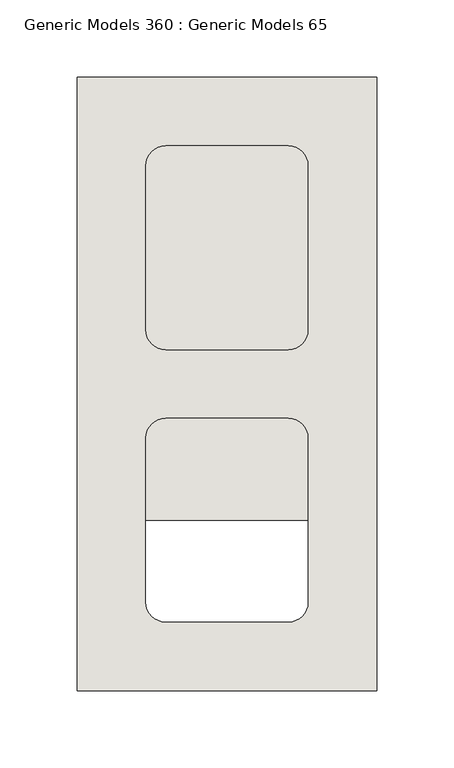
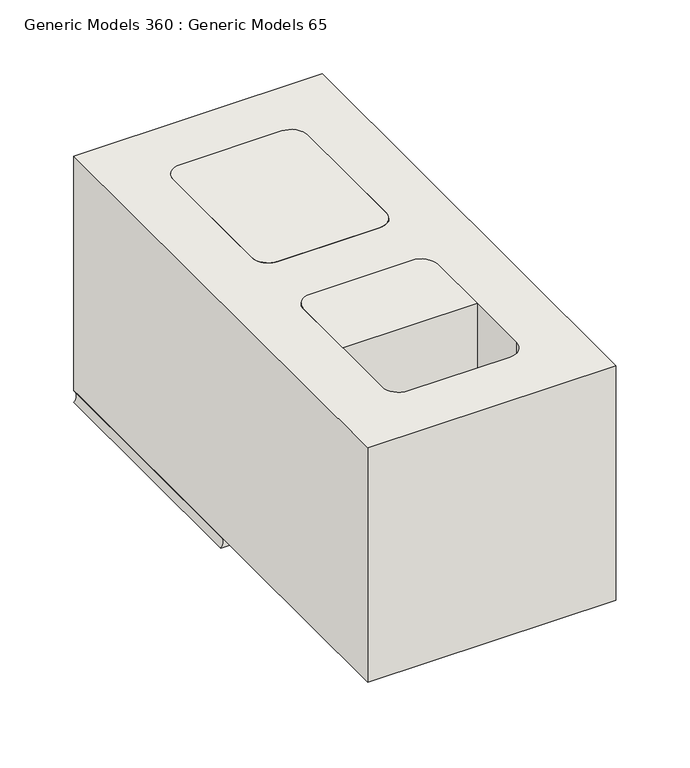
"""IFC4 building model written with IfcOpenShell, lengths in millimetres: wall geometry, Generic Models 360 : Generic Models 65."""

from ifc_helpers import new_model, si_unit, point, frame, frame_2d, origin, place, context, project, spatial, polyline, circle_curve, trimmed, segment, composite_curve, outline, extrude, source, transform, mapped, element, save
from ifc_brep_helpers import plane_surface, revolved_surface, advanced_brep


def generic_models_360_generic_models_65_2d37a0e6(model_context):
    return source(origin(), model_context, "Body", "SolidModel", [
        advanced_brep(
        [(430198.2125, 503.2375, 822.325), (430004.5375, 503.2375, 822.325), (430004.5375, 503.2375, 812.8), (430198.2125, 503.2375, 812.8), (430198.2125, 701.675, 822.325), (430198.2125, 701.675, 812.8), (430004.5375, 701.675, 812.8), (430004.5375, 701.675, 822.325), (430153.7625, 538.1625, 822.325), (430141.0625, 525.4625, 822.325), (430061.6875, 525.4625, 822.325), (430048.9875, 538.1625, 822.325), (430048.9875, 644.525, 822.325), (430061.6875, 657.225, 822.325), (430141.0625, 657.225, 822.325), (430153.7625, 644.525, 822.325), (430141.0625, 525.4625, 812.8), (430153.7625, 538.1625, 812.8), (430061.6875, 525.4625, 812.8), (430048.9875, 538.1625, 812.8), (430048.9875, 644.525, 812.8), (430061.6875, 657.225, 812.8), (430141.0625, 657.225, 812.8), (430153.7625, 644.525, 812.8)],
        [
            (0, 1),
            (1, 2, circle_curve(frame((429999.6545028, 503.2375, 817.5625), z_axis=(0.0, 1.0, 0.0), x_axis=(1.0, 0.0, 0.0)), 6.8209287)),
            (2, 3),
            (3, 0, circle_curve(frame((430203.0954972, 503.2375, 817.5625), z_axis=(0.0, 1.0, 0.0), x_axis=(-1.0, 0.0, 0.0)), 6.8209287)),
            (4, 5, circle_curve(frame((430203.0954972, 701.675, 817.5625), z_axis=(0.0, -1.0, 0.0), x_axis=(-1.0, 0.0, 0.0)), 6.8209287)),
            (5, 6),
            (6, 7, circle_curve(frame((429999.6545028, 701.675, 817.5625), z_axis=(0.0, -1.0, 0.0), x_axis=(1.0, 0.0, 0.0)), 6.8209287)),
            (7, 4),
            (0, 4),
            (7, 1),
            (8, 9, circle_curve(frame((430141.0625, 538.1625, 822.325), z_axis=(0.0, 0.0, -1.0), x_axis=(-1.0, 0.0, 0.0)), 12.7)),
            (9, 10),
            (10, 11, circle_curve(frame((430061.6875, 538.1625, 822.325), z_axis=(0.0, 0.0, -1.0), x_axis=(-1.0, 0.0, 0.0)), 12.7)),
            (11, 12),
            (12, 13, circle_curve(frame((430061.6875, 644.525, 822.325), z_axis=(0.0, 0.0, -1.0), x_axis=(-1.0, 0.0, 0.0)), 12.7)),
            (13, 14),
            (14, 15, circle_curve(frame((430141.0625, 644.525, 822.325), z_axis=(0.0, 0.0, -1.0), x_axis=(-1.0, 0.0, 0.0)), 12.7)),
            (15, 8),
            (16, 9),
            (8, 17),
            (17, 16, circle_curve(frame((430141.0625, 538.1625, 812.8), z_axis=(0.0, 0.0, -1.0), x_axis=(-1.0, 0.0, 0.0)), 12.7)),
            (16, 18),
            (18, 10),
            (18, 19, circle_curve(frame((430061.6875, 538.1625, 812.8), z_axis=(0.0, 0.0, -1.0), x_axis=(-1.0, 0.0, 0.0)), 12.7)),
            (19, 11),
            (19, 20),
            (20, 12),
            (20, 21, circle_curve(frame((430061.6875, 644.525, 812.8), z_axis=(0.0, 0.0, -1.0), x_axis=(-1.0, 0.0, 0.0)), 12.7)),
            (21, 13),
            (21, 22),
            (22, 14),
            (22, 23, circle_curve(frame((430141.0625, 644.525, 812.8), z_axis=(0.0, 0.0, -1.0), x_axis=(-1.0, 0.0, 0.0)), 12.7)),
            (23, 15),
            (23, 17),
            (6, 2),
            (5, 3),
        ],
        [
            plane_surface(frame((430101.375, 503.2375, 822.721875), z_axis=(0.0, -1.0, 0.0), x_axis=(0.0, 0.0, 1.0))),
            plane_surface(frame((430101.375, 701.675, 822.721875), z_axis=(0.0, 1.0, 0.0), x_axis=(0.0, 0.0, 1.0))),
            plane_surface(frame((430198.2125, 503.2375, 822.325), z_axis=(0.0, 0.0, 1.0), x_axis=(0.0, 1.0, 0.0))),
            revolved_surface(polyline([(430128.3625, 538.1625, 822.325), (430128.3625, 538.1625, 812.8)]), (430141.0625, 538.1625, 1006.475), (0.0, 0.0, 1.0)),
            plane_surface(frame((430061.6875, 525.4625, 1006.475), z_axis=(0.0, 1.0, 0.0), x_axis=(0.0, 0.0, -1.0))),
            revolved_surface(polyline([(430048.9875, 538.1625, 822.325), (430048.9875, 538.1625, 812.8)]), (430061.6875, 538.1625, 1006.475), (0.0, 0.0, 1.0)),
            plane_surface(frame((430048.9875, 644.525, 1006.475), z_axis=(1.0, 0.0, 0.0), x_axis=(0.0, 0.0, -1.0))),
            revolved_surface(polyline([(430048.9875, 644.525, 822.325), (430048.9875, 644.525, 812.8)]), (430061.6875, 644.525, 1006.475), (0.0, 0.0, 1.0)),
            plane_surface(frame((430141.0625, 657.225, 1006.475), z_axis=(0.0, -1.0, 0.0), x_axis=(0.0, 0.0, -1.0))),
            revolved_surface(polyline([(430128.3625, 644.525, 822.325), (430128.3625, 644.525, 812.8)]), (430141.0625, 644.525, 1006.475), (0.0, 0.0, 1.0)),
            plane_surface(frame((430153.7625, 538.1625, 1006.475), z_axis=(-1.0, 0.0, 0.0), x_axis=(0.0, 0.0, -1.0))),
            revolved_surface(polyline([(430006.4754315, 701.675, 817.5625), (430006.4754315, 503.2375, 817.5625)]), (429999.6545028, 503.2375, 817.5625), (0.0, 1.0, 0.0)),
            plane_surface(frame((430004.5375, 503.2375, 812.8), z_axis=(0.0, 0.0, -1.0), x_axis=(0.0, 1.0, 0.0))),
            revolved_surface(polyline([(430196.2745685, 701.675, 817.5625), (430196.2745685, 503.2375, 817.5625)]), (430203.0954972, 503.2375, 817.5625), (0.0, 1.0, 0.0)),
        ],
        [
            (0, [[1, 2, 3, 4]]),
            (1, [[5, 6, 7, 8]]),
            (2, [[-1, 9, -8, 10], [11, 12, 13, 14, 15, 16, 17, 18]]),
            (3, [[19, -11, 20, 21]]),
            (4, [[-19, 22, 23, -12]]),
            (5, [[-23, 24, 25, -13]]),
            (6, [[-25, 26, 27, -14]]),
            (7, [[-27, 28, 29, -15]]),
            (8, [[-29, 30, 31, -16]]),
            (9, [[-31, 32, 33, -17]]),
            (10, [[-33, 34, -20, -18]]),
            (11, [[-2, -10, -7, 35]]),
            (12, [[-3, -35, -6, 36], [-21, -34, -32, -30, -28, -26, -24, -22]]),
            (13, [[-4, -36, -5, -9]]),
        ],
    ),
        extrude(outline(composite_curve([segment(trimmed(circle_curve(frame_2d((430141.0625, 538.1625)), 12.7), [point((430153.7625, 538.1625))], [point((430141.0625, 525.4625))], False, "CARTESIAN"), True, "CONTINUOUS"), segment(polyline([(430141.0625, 525.4625), (430061.6875, 525.4625)]), True, "CONTINUOUS"), segment(trimmed(circle_curve(frame_2d((430061.6875, 538.1625)), 12.7), [point((430061.6875, 525.4625))], [point((430048.9875, 538.1625))], False, "CARTESIAN"), True, "CONTINUOUS"), segment(polyline([(430048.9875, 538.1625), (430048.9875, 644.525)]), True, "CONTINUOUS"), segment(trimmed(circle_curve(frame_2d((430061.6875, 644.525)), 12.7), [point((430048.9875, 644.525))], [point((430061.6875, 657.225))], False, "CARTESIAN"), True, "CONTINUOUS"), segment(polyline([(430061.6875, 657.225), (430141.0625, 657.225)]), True, "CONTINUOUS"), segment(trimmed(circle_curve(frame_2d((430141.0625, 644.525)), 12.7), [point((430141.0625, 657.225))], [point((430153.7625, 644.525))], False, "CARTESIAN"), True, "CONTINUOUS"), segment(polyline([(430153.7625, 644.525), (430153.7625, 538.1625)]), True, "CONTINUOUS")], self_intersect=False)), frame((0.0, 0.0, 812.8), z_axis=(0.0, 0.0, 1.0), x_axis=(1.0, 0.0, 0.0)), (0.0, 0.0, 1.0), 203.2),
        extrude(outline(composite_curve([segment(trimmed(circle_curve(frame_2d((430061.6875, 468.3125)), 12.7), [point((430048.9875, 468.3125))], [point((430061.6875, 481.0125))], False, "CARTESIAN"), True, "CONTINUOUS"), segment(polyline([(430061.6875, 481.0125), (430141.0625, 481.0125)]), True, "CONTINUOUS"), segment(trimmed(circle_curve(frame_2d((430141.0625, 468.3125)), 12.7), [point((430141.0625, 481.0125))], [point((430153.7625, 468.3125))], False, "CARTESIAN"), True, "CONTINUOUS"), segment(polyline([(430153.7625, 468.3125), (430153.7625, 415.13125), (430048.9875, 415.13125), (430048.9875, 468.3125)]), True, "CONTINUOUS")], self_intersect=False)), frame((0.0, 0.0, 812.8), z_axis=(0.0, 0.0, 1.0), x_axis=(1.0, 0.0, 0.0)), (0.0, 0.0, 1.0), 203.2),
        extrude(outline(polyline([(430198.2125, 304.8), (430004.5375, 304.8), (430004.5375, 701.675), (430198.2125, 701.675), (430198.2125, 304.8)]), holes=[composite_curve([segment(polyline([(430153.7625, 538.1625), (430153.7625, 644.525)]), True, "CONTINUOUS"), segment(trimmed(circle_curve(frame_2d((430141.0625, 644.525)), 12.7), [point((430153.7625, 644.525))], [point((430141.0625, 657.225))], True, "CARTESIAN"), True, "CONTINUOUS"), segment(polyline([(430141.0625, 657.225), (430061.6875, 657.225)]), True, "CONTINUOUS"), segment(trimmed(circle_curve(frame_2d((430061.6875, 644.525)), 12.7), [point((430061.6875, 657.225))], [point((430048.9875, 644.525))], True, "CARTESIAN"), True, "CONTINUOUS"), segment(polyline([(430048.9875, 644.525), (430048.9875, 538.1625)]), True, "CONTINUOUS"), segment(trimmed(circle_curve(frame_2d((430061.6875, 538.1625)), 12.7), [point((430048.9875, 538.1625))], [point((430061.6875, 525.4625))], True, "CARTESIAN"), True, "CONTINUOUS"), segment(polyline([(430061.6875, 525.4625), (430141.0625, 525.4625)]), True, "CONTINUOUS"), segment(trimmed(circle_curve(frame_2d((430141.0625, 538.1625)), 12.7), [point((430141.0625, 525.4625))], [point((430153.7625, 538.1625))], True, "CARTESIAN"), True, "CONTINUOUS")], self_intersect=False), composite_curve([segment(polyline([(430048.9875, 468.3125), (430048.9875, 361.95)]), True, "CONTINUOUS"), segment(trimmed(circle_curve(frame_2d((430061.6875, 361.95)), 12.7), [point((430048.9875, 361.95))], [point((430061.6875, 349.25))], True, "CARTESIAN"), True, "CONTINUOUS"), segment(polyline([(430061.6875, 349.25), (430141.0625, 349.25)]), True, "CONTINUOUS"), segment(trimmed(circle_curve(frame_2d((430141.0625, 361.95)), 12.7), [point((430141.0625, 349.25))], [point((430153.7625, 361.95))], True, "CARTESIAN"), True, "CONTINUOUS"), segment(polyline([(430153.7625, 361.95), (430153.7625, 468.3125)]), True, "CONTINUOUS"), segment(trimmed(circle_curve(frame_2d((430141.0625, 468.3125)), 12.7), [point((430153.7625, 468.3125))], [point((430141.0625, 481.0125))], True, "CARTESIAN"), True, "CONTINUOUS"), segment(polyline([(430141.0625, 481.0125), (430061.6875, 481.0125)]), True, "CONTINUOUS"), segment(trimmed(circle_curve(frame_2d((430061.6875, 468.3125)), 12.7), [point((430061.6875, 481.0125))], [point((430048.9875, 468.3125))], True, "CARTESIAN"), True, "CONTINUOUS")], self_intersect=False)]), frame((0.0, 0.0, 822.325), z_axis=(0.0, 0.0, 1.0), x_axis=(1.0, 0.0, 0.0)), (0.0, 0.0, 1.0), 193.675),
    ])


if __name__ == "__main__":
    model = new_model("IFC4")
    model_context = context("Model", 3, world=origin())
    ifc_project = project(units=[si_unit("LENGTHUNIT", "METRE", prefix="MILLI")], contexts=[model_context])
    site = spatial("IfcSite", under=ifc_project)
    building = spatial("IfcBuilding", under=site)
    placement = place(None, origin())
    generic_models_360_generic_models_65_shape = generic_models_360_generic_models_65_2d37a0e6(model_context)
    element("IfcWall", 1, ObjectType="Generic Models 360 : Generic Models 65", at=placement, inside=building, context=model_context, shape_type="MappedRepresentation", body=[
        mapped(generic_models_360_generic_models_65_shape, transform((0.0, 0.0, 0.0), x_axis=(1.0, 0.0, 0.0), y_axis=(0.0, 1.0, 0.0), z_axis=(0.0, 0.0, 1.0))),
    ])
    save(model, "model.ifc")

# Revit data of these elements
# Element 1 (IfcWall, "Generic Models 360 : Generic Models 65")
#   Materials on its faces: "CMU (SEE 'WALL TAG' FOR SIZE)", "FILL CORE IF APPLICABLE - SEE STRUCTURAL DWGS FOR DETAILS", "MORTAR JOINT"
# Materials
#   "CMU (SEE 'WALL TAG' FOR SIZE)": class "Masonry", colour RGB 203 203 199, transparency 0, Description = "Concrete masonry units", Cost = 0
#   "FILL CORE IF APPLICABLE - SEE STRUCTURAL DWGS FOR DETAILS": class "Generic", colour RGB 170 170 170, transparency 0, Cost = 0
#   "MORTAR JOINT": class "Generic", colour RGB 120 120 120, transparency 0, Cost = 0
